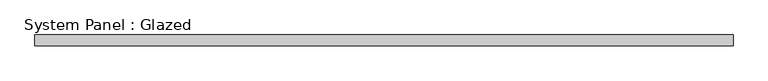
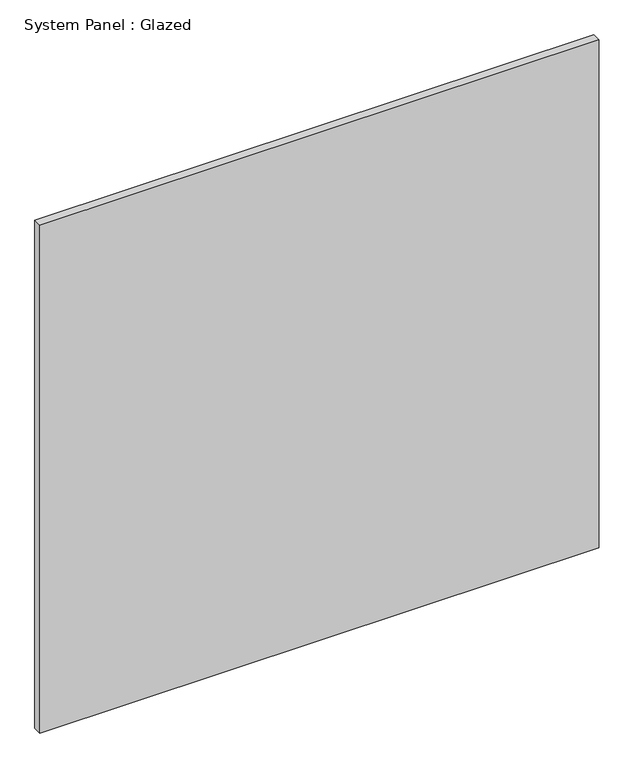
"""IFC4 building model written with IfcOpenShell, lengths in millimetres: plate geometry, System Panel : Glazed."""

from ifc_helpers import new_model, si_unit, origin, origin_with_axes, place, context, project, spatial, polyline, outline, extrude, source, transform, mapped, element, save


def system_panel_glazed_619493b4(model_context):
    return source(origin(), model_context, "Body", "SweptSolid", [
        extrude(outline(polyline([(807.5, 24.5), (-807.5, 24.5), (-807.5, 49.5), (807.5, 49.5), (807.5, 24.5)])), origin_with_axes(), (0.0, 0.0, 1.0), 1550.0),
    ])


if __name__ == "__main__":
    model = new_model("IFC4")
    model_context = context("Model", 3, world=origin())
    ifc_project = project(units=[si_unit("LENGTHUNIT", "METRE", prefix="MILLI")], contexts=[model_context])
    site = spatial("IfcSite", under=ifc_project)
    building = spatial("IfcBuilding", under=site)
    placement = place(None, origin())
    system_panel_glazed_shape = system_panel_glazed_619493b4(model_context)
    element("IfcPlate", 1, ObjectType="System Panel : Glazed", at=placement, inside=building, context=model_context, shape_type="MappedRepresentation", body=[
        mapped(system_panel_glazed_shape, transform((0.0, 0.0, 0.0), x_axis=(1.0, 0.0, 0.0), y_axis=(0.0, 1.0, 0.0), z_axis=(0.0, 0.0, 1.0))),
    ])
    save(model, "model.ifc")

# Revit data of these elements
# Element 1 (IfcPlate, "System Panel : Glazed")
#   Materials on its faces: "Glass"
# Materials
#   "Glass": class "Glass", colour RGB 0 128 192, transparency 0.9
